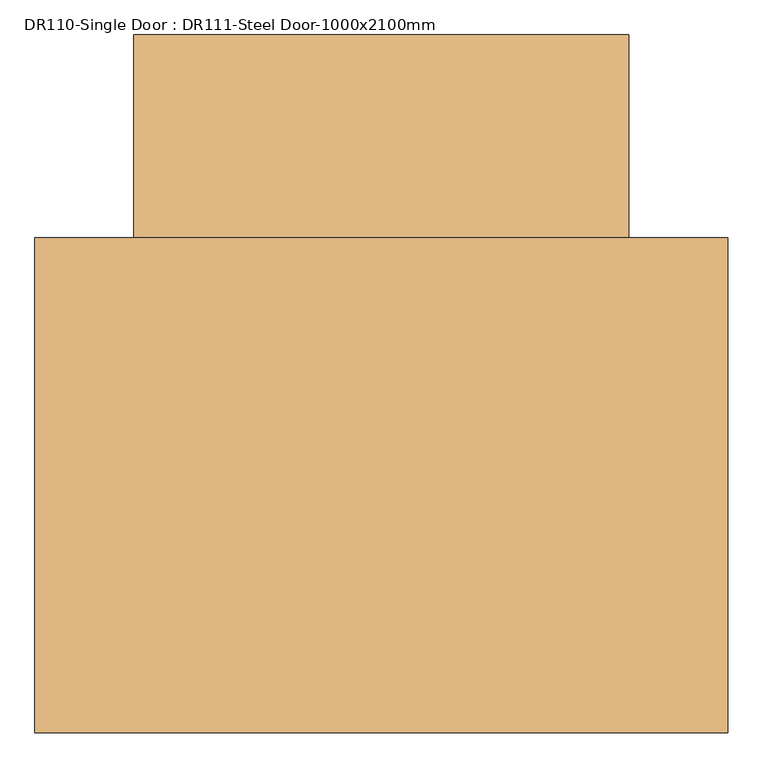
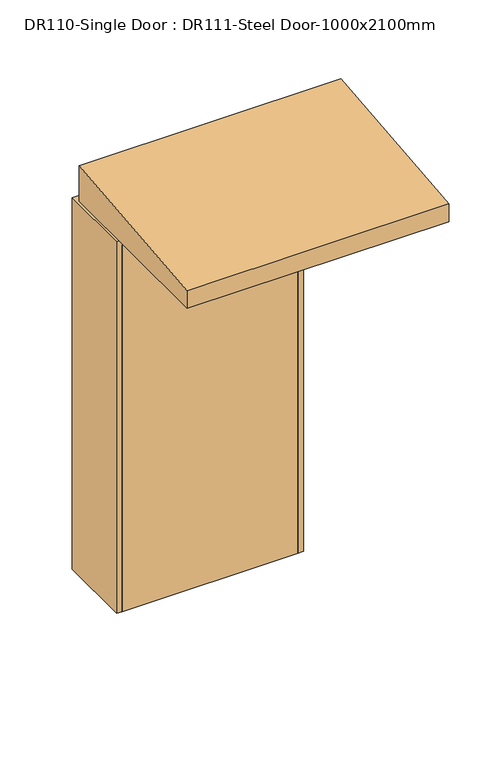
"""IFC4 building model written with IfcOpenShell, lengths in millimetres: door geometry, DR110-Single Door : DR111-Steel Door-1000x2100mm."""

from ifc_helpers import new_model, si_unit, frame, origin, origin_with_axes, place, context, project, spatial, polyline, outline, extrude, faceted_brep, source, transform, mapped, element, save


def dr110_single_door_dr111_steel_door_1000x2100mm_4484fb18(model_context):
    return source(origin(), model_context, "Body", "SolidModel", [
        extrude(outline(polyline([(470.0, -205.0), (-470.0, -205.0), (-470.0, -170.0), (470.0, -170.0), (470.0, -205.0)])), origin_with_axes(), (0.0, 0.0, 1.0), 2070.0),
        faceted_brep([(470.0, -205.0, 0.0), (470.0, -170.0, 0.0), (450.0, -170.0, 0.0), (450.0, 170.0, 0.0), (470.0, 170.0, 0.0), (470.0, 205.0, 0.0), (500.0, 205.0, 0.0), (500.0, -205.0, 0.0), (500.0, -205.0, 2100.0), (-500.0, -205.0, 2100.0), (-500.0, -205.0, 0.0), (-470.0, -205.0, 0.0), (-470.0, -205.0, 2070.0), (470.0, -205.0, 2070.0), (500.0, 205.0, 2100.0), (470.0, 205.0, 2070.0), (-470.0, 205.0, 2070.0), (-470.0, 205.0, 0.0), (-500.0, 205.0, 0.0), (-500.0, 205.0, 2100.0), (470.0, 170.0, 2070.0), (450.0, 170.0, 2050.0), (-450.0, 170.0, 2050.0), (-450.0, 170.0, 0.0), (-470.0, 170.0, 0.0), (-470.0, 170.0, 2070.0), (450.0, -170.0, 2050.0), (470.0, -170.0, 2070.0), (-470.0, -170.0, 2070.0), (-470.0, -170.0, 0.0), (-450.0, -170.0, 0.0), (-450.0, -170.0, 2050.0)], [[[0, 1, 2, 3, 4, 5, 6, 7]], [[7, 8, 9, 10, 11, 12, 13, 0]], [[6, 14, 8, 7]], [[5, 15, 16, 17, 18, 19, 14, 6]], [[4, 20, 15, 5]], [[3, 21, 22, 23, 24, 25, 20, 4]], [[2, 26, 21, 3]], [[1, 27, 28, 29, 30, 31, 26, 2]], [[0, 13, 27, 1]], [[12, 11, 29, 28]], [[11, 10, 18, 17, 24, 23, 30, 29]], [[19, 18, 10, 9]], [[25, 24, 17, 16]], [[31, 30, 23, 22]], [[14, 19, 9, 8]], [[20, 25, 16, 15]], [[26, 31, 22, 21]], [[13, 12, 28, 27]]]),
        extrude(outline(polyline([(-1205.0, 2400.0), (-1205.0, 2500.0), (-205.0, 2600.0), (-205.0, 2400.0), (-1205.0, 2400.0)])), frame((-700.0, 0.0, 0.0), z_axis=(1.0, 0.0, 0.0), x_axis=(0.0, 1.0, 0.0)), (0.0, 0.0, 1.0), 1400.0),
    ])


if __name__ == "__main__":
    model = new_model("IFC4")
    model_context = context("Model", 3, world=origin())
    ifc_project = project(units=[si_unit("LENGTHUNIT", "METRE", prefix="MILLI")], contexts=[model_context])
    site = spatial("IfcSite", under=ifc_project)
    building = spatial("IfcBuilding", under=site)
    placement = place(None, origin())
    dr110_single_door_dr111_steel_door_1000x2100mm_shape = dr110_single_door_dr111_steel_door_1000x2100mm_4484fb18(model_context)
    element("IfcDoor", 1, ObjectType="DR110-Single Door : DR111-Steel Door-1000x2100mm", at=placement, inside=building, context=model_context, shape_type="MappedRepresentation", body=[
        mapped(dr110_single_door_dr111_steel_door_1000x2100mm_shape, transform((0.0, 0.0, 0.0), x_axis=(1.0, 0.0, 0.0), y_axis=(0.0, 1.0, 0.0), z_axis=(0.0, 0.0, 1.0))),
    ])
    save(model, "model.ifc")

# Revit data of these elements
# Type "DR110-Single Door : DR111-Steel Door-1000x2100mm"
#   Type Mark = "SD"
#   Analytic Construction = "<None>"
#   프레임 투영 외부. = 25 mm
#   프레임 투영 내부. = 25 mm
#   프레임 폭 = 75 mm
#   Height = 2100 mm
#   Width = 1000 mm
#   Define Thermal Properties by = 1
#   Canopy [instance default] = yes
#   문 패널 = SD1 문 패널
#   문 프레임 = A04AQ098-00002_Steel Door_non FP_single
#   Function = (empty or 0)
#   Wall Closure = (empty or 0)
# Element 1 (IfcDoor, "DR110-Single Door : DR111-Steel Door-1000x2100mm")
#   Materials on its faces: "A04AQ098-00002_Steel Door_non FP_single", "SD1 문 패널"
# Materials
#   "SD1 문 패널": class "금속", colour RGB 247 247 247, transparency 0
#   "A04AQ098-00002_Steel Door_non FP_single": class "금속", colour RGB 247 247 247, transparency 0, Description = "Steel Door", W00) Work Master Code = "A04AQ098-00002", W01) Work Master_Lv1 = "Finishing Work", W02) Work Master_Lv2 = "Door & Window Work", W03) Work Master_Spec.1 = "Steel Door w/ Steel Frame", W04) Work Master_Spec.2 = "Fire Protective Rating: N/A, Single Door", W05) Work Master_Spec.3 = "w/ Hardware & Accessories", Cost = 0
